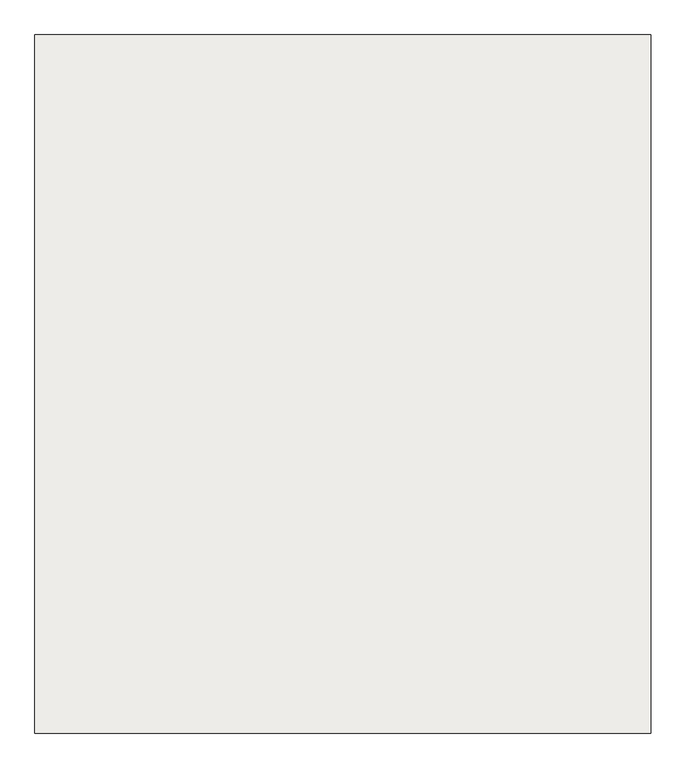
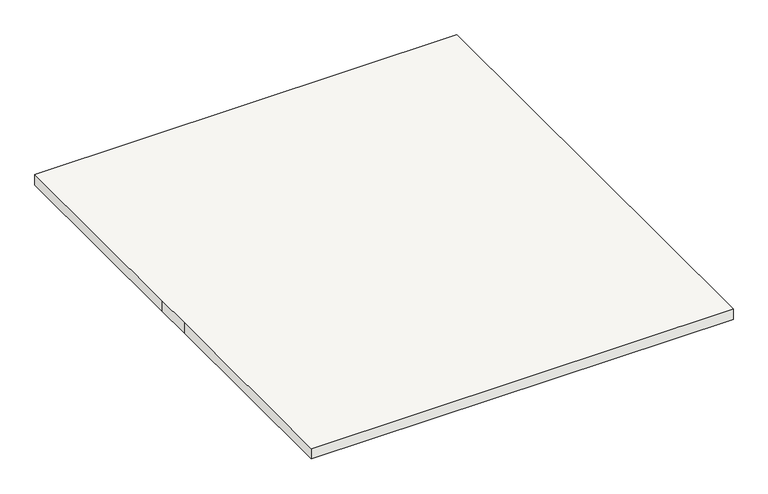
"""IFC4 building model written with IfcOpenShell, lengths in millimetres: slab geometry."""

import ifcopenshell
import ifcopenshell.guid

model = None  # the IFC model being written
_history = None  # IfcOwnerHistory: only IFC2X3 demands one
_inside = {}  # id of a spatial element -> (the spatial element, [elements in it])
_under = {}  # id of a project, library or spatial element -> (it, [spatial elements below it])
_declared = {}  # id of a project -> (the project, [libraries it declares])
_typed = {}  # id of a type object -> (the type object, [elements of that type])
_made_of = {}  # id of a material, layer set ... -> (it, [elements and type objects made of it])


def new_model(schema):
    """Start an empty IFC model of exactly this schema.

    Asked for "IFC4X3", IfcOpenShell would pick the latest addendum, in which some entities
    have other attributes; the version numbers below select the first issue.
    IFC2X3 requires an IfcOwnerHistory on every rooted entity: one is made here for all.
    """
    global model, _history
    if schema == "IFC4X3":
        model = ifcopenshell.file(schema_version=(4, 3, 0, 0))
    else:
        model = ifcopenshell.file(schema=schema)
    _inside.clear()
    _under.clear()
    _declared.clear()
    _typed.clear()
    _made_of.clear()
    _history = None
    if model.schema == "IFC2X3":
        org = make("IfcOrganization", Name="unknown")
        user = make(
            "IfcPersonAndOrganization",
            ThePerson=make("IfcPerson", FamilyName="unknown"),
            TheOrganization=org,
        )
        app = make(
            "IfcApplication",
            ApplicationDeveloper=org,
            Version="unknown",
            ApplicationFullName="unknown",
            ApplicationIdentifier="unknown",
        )
        _history = make(
            "IfcOwnerHistory",
            OwningUser=user,
            OwningApplication=app,
            ChangeAction="ADDED",
            CreationDate=0,
        )
    return model


def make(cls, **values):
    """One entity of the class cls with the attributes given. An attribute that is None is left unset."""
    return model.create_entity(
        cls, **{name: value for name, value in values.items() if value is not None}
    )


def rooted(cls, **values):
    """An entity with a GlobalId (a new one), such as an element, a storey or a relation."""
    return make(cls, GlobalId=ifcopenshell.guid.new(), OwnerHistory=_history, **values)


def si_unit(unit_type, name, prefix=None):
    """IfcSIUnit, for example si_unit("LENGTHUNIT", "METRE", prefix="MILLI")."""
    return make("IfcSIUnit", UnitType=unit_type, Prefix=prefix, Name=name)


def assignment(units):
    """IfcUnitAssignment: the units of a project."""
    return None if units is None else make("IfcUnitAssignment", Units=units)


def point(xyz):
    """IfcCartesianPoint."""
    return None if xyz is None else make("IfcCartesianPoint", Coordinates=xyz)


def direction(xyz):
    """IfcDirection."""
    return None if xyz is None else make("IfcDirection", DirectionRatios=xyz)


def frame(location, z_axis=None, x_axis=None):
    """IfcAxis2Placement3D, a coordinate frame: its origin and axes. An axis left out is left unset."""
    return make(
        "IfcAxis2Placement3D",
        Location=point(location),
        Axis=direction(z_axis),
        RefDirection=direction(x_axis),
    )


def origin():
    """The frame at (0, 0, 0) with its axes left unset."""
    return frame((0.0, 0.0, 0.0))


def place(relative_to, where):
    """IfcLocalPlacement: puts the frame where relative to a parent placement (None: the world)."""
    return make(
        "IfcLocalPlacement", PlacementRelTo=relative_to, RelativePlacement=where
    )


def context(
    kind, dimensions, precision=None, world=None, true_north=None, identifier=None
):
    """IfcGeometricRepresentationContext, for example the 3D "Model" context."""
    return make(
        "IfcGeometricRepresentationContext",
        ContextIdentifier=identifier,
        ContextType=kind,
        CoordinateSpaceDimension=dimensions,
        Precision=precision,
        WorldCoordinateSystem=world,
        TrueNorth=true_north,
    )


def project(units=None, contexts=None):
    """IfcProject with its units and contexts."""
    return rooted(
        "IfcProject",
        Name="project",
        RepresentationContexts=contexts,
        UnitsInContext=assignment(units),
    )


def spatial(cls, under=None, at=None, **own):
    """A site, building, storey or space (cls), placed at a placement, below another one or the project."""
    s = rooted(cls, ObjectPlacement=at, **own)
    if under is not None:
        _under.setdefault(under.id(), (under, []))[1].append(s)
    return s


def polyline(points):
    """IfcPolyline through the points."""
    return make("IfcPolyline", Points=[point(p) for p in points])


def outline(outer, holes=None, kind="AREA"):
    """IfcArbitraryClosedProfileDef: a profile drawn as a closed curve; with holes, ...WithVoids."""
    if holes is None:
        return make("IfcArbitraryClosedProfileDef", ProfileType=kind, OuterCurve=outer)
    return make(
        "IfcArbitraryProfileDefWithVoids",
        ProfileType=kind,
        OuterCurve=outer,
        InnerCurves=holes,
    )


def extrude(swept, where, along, depth):
    """IfcExtrudedAreaSolid: the profile swept, set in the frame where, extruded along a direction by depth."""
    return make(
        "IfcExtrudedAreaSolid",
        SweptArea=swept,
        Position=where,
        ExtrudedDirection=direction(along),
        Depth=depth,
    )


def shape(context_of_items, identifier, shape_type, items):
    """IfcShapeRepresentation: the items that make up one representation, for example the "Body"."""
    return make(
        "IfcShapeRepresentation",
        ContextOfItems=context_of_items,
        RepresentationIdentifier=identifier,
        RepresentationType=shape_type,
        Items=items,
    )


def source(mapping_origin, context_of_items, identifier, shape_type, items):
    """IfcRepresentationMap: a shape defined once, which mapped items show again and again."""
    return make(
        "IfcRepresentationMap",
        MappingOrigin=mapping_origin,
        MappedRepresentation=shape(context_of_items, identifier, shape_type, items),
    )


def transform(
    local_origin,
    x_axis=None,
    y_axis=None,
    z_axis=None,
    scale=None,
    scale2=None,
    scale3=None,
    uniform=True,
):
    """IfcCartesianTransformationOperator3D, or its non-uniform kind. x_axis, y_axis, z_axis: its Axis1, 2, 3."""
    if uniform:
        return make(
            "IfcCartesianTransformationOperator3D",
            Axis1=direction(x_axis),
            Axis2=direction(y_axis),
            LocalOrigin=point(local_origin),
            Scale=scale,
            Axis3=direction(z_axis),
        )
    return make(
        "IfcCartesianTransformationOperator3DnonUniform",
        Axis1=direction(x_axis),
        Axis2=direction(y_axis),
        LocalOrigin=point(local_origin),
        Scale=scale,
        Axis3=direction(z_axis),
        Scale2=scale2,
        Scale3=scale3,
    )


def mapped(mapping_source, mapping_target):
    """IfcMappedItem: shows the shape of a source again, moved by a transform."""
    return make(
        "IfcMappedItem", MappingSource=mapping_source, MappingTarget=mapping_target
    )


def made_of(thing, what):
    """Note that an element or type object is made of a material, layer set ...; save() writes the relation."""
    if what is not None:
        _made_of.setdefault(what.id(), (what, []))[1].append(thing)
    return thing


def element(
    cls,
    number,
    at=None,
    inside=None,
    cuts=None,
    type_object=None,
    material=None,
    context=None,
    identifier="Body",
    shape_type=None,
    held_by="IfcProductDefinitionShape",
    body=None,
    shapes=None,
    **own,
):
    """One element of the class cls, such as IfcWall. Its Tag is "e" and its number.

    at: its placement. inside: the storey or other place that contains it. cuts: it is an
    opening in that element (IfcRelVoidsElement). A single representation is given by context,
    identifier, shape_type and body (its items); several are given by shapes. held_by: the class
    of the entity that holds the representations. save() writes the other relations.
    """
    e = rooted(cls, Tag="e%d" % number, ObjectPlacement=at, **own)
    if body is not None:
        shapes = [shape(context, identifier, shape_type, body)]
    if shapes is not None:
        e.Representation = make(held_by, Representations=shapes)
    if inside is not None:
        _inside.setdefault(inside.id(), (inside, []))[1].append(e)
    if cuts is not None:
        rooted(
            "IfcRelVoidsElement", RelatingBuildingElement=cuts, RelatedOpeningElement=e
        )
    if type_object is not None:
        _typed.setdefault(type_object.id(), (type_object, []))[1].append(e)
    return made_of(e, material)


def aggregate(whole, parts):
    """IfcRelAggregates: a whole, such as a stair, and the parts it consists of."""
    return rooted("IfcRelAggregates", RelatingObject=whole, RelatedObjects=parts)


def save(model, path):
    """Write the relations noted so far, then the file.

    IfcRelAggregates (storeys below a building ...), IfcRelContainedInSpatialStructure (elements
    in a storey), IfcRelDefinesByType, IfcRelAssociatesMaterial and IfcRelDeclares: one each for
    every whole, place, type object, material and project.
    """
    for whole, parts in _under.values():
        aggregate(whole, parts)
    for where, things in _inside.values():
        rooted(
            "IfcRelContainedInSpatialStructure",
            RelatedElements=things,
            RelatingStructure=where,
        )
    for kind, things in _typed.values():
        rooted("IfcRelDefinesByType", RelatedObjects=things, RelatingType=kind)
    for what, things in _made_of.values():
        rooted("IfcRelAssociatesMaterial", RelatedObjects=things, RelatingMaterial=what)
    for by, libraries in _declared.values():
        rooted("IfcRelDeclares", RelatingContext=by, RelatedDefinitions=libraries)
    model.write(path)


def slab_0549d9b8(model_context):
    return source(origin(), model_context, "Body", "SweptSolid", [
        extrude(outline(polyline([(5276.5556606, 3685.7983707), (7194.8909543, 3685.7983707), (7194.8909543, 1510.81281), (5276.5556606, 1510.81281), (5276.5556606, 2510.81281), (5276.5556606, 2685.7983707), (5276.5556606, 3685.7983707)])), frame((0.0, 0.0, 4750.0), z_axis=(0.0, 0.0, 1.0), x_axis=(1.0, 0.0, 0.0)), (0.0, 0.0, 1.0), 50.0),
    ])


if __name__ == "__main__":
    model = new_model("IFC4")
    model_context = context("Model", 3, world=origin())
    ifc_project = project(units=[si_unit("LENGTHUNIT", "METRE", prefix="MILLI")], contexts=[model_context])
    site = spatial("IfcSite", under=ifc_project)
    building = spatial("IfcBuilding", under=site)
    placement = place(None, origin())
    slab_shape = slab_0549d9b8(model_context)
    element("IfcSlab", 1, at=placement, inside=building, context=model_context, shape_type="MappedRepresentation", body=[
        mapped(slab_shape, transform((0.0, 0.0, 0.0), x_axis=(1.0, 0.0, 0.0), y_axis=(0.0, 1.0, 0.0), z_axis=(0.0, 0.0, 1.0))),
    ])
    save(model, "model.ifc")
